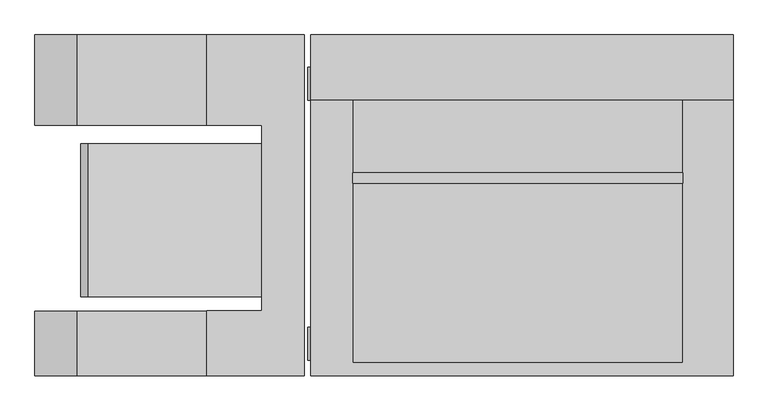
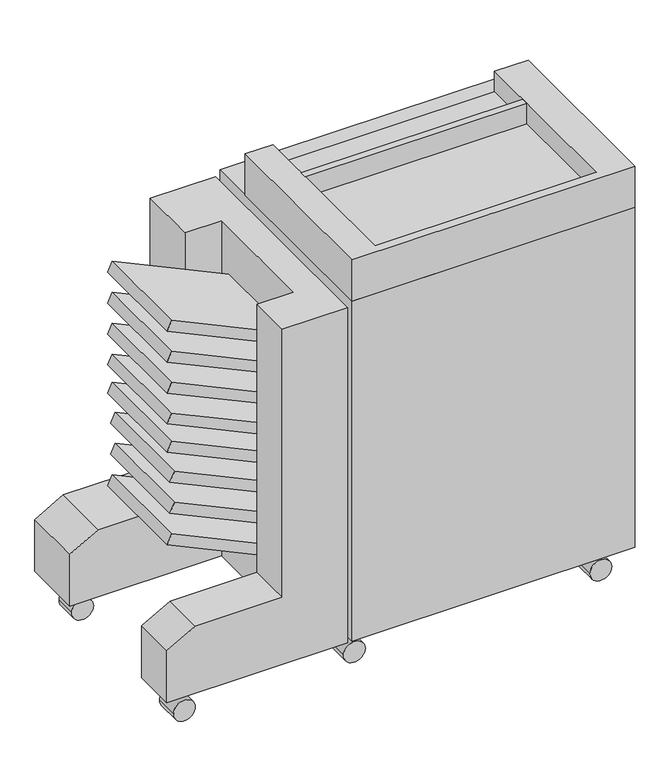
"""IFC4 building model written with IfcOpenShell, lengths in millimetres: proxy geometry, Kopierer : Kopierer."""

from ifc_helpers import new_model, si_unit, point, frame, frame_2d, origin, place, context, project, spatial, polyline, circle_curve, trimmed, segment, composite_curve, outline, extrude, faceted_brep, source, transform, mapped, element, save


def specialty_equipment_65fc0428(model_context):
    return source(origin(), model_context, "Body", "SolidModel", [
        extrude(outline(polyline([(387.7567294, -681.6535349), (364.7365116, -692.3880388), (232.9041289, -409.6725817), (260.929928, -409.6725817), (387.7567294, -681.6535349)])), frame((0.0, -167.6536807, 0.0), z_axis=(0.0, 1.0, 0.0), x_axis=(0.0, 0.0, 1.0)), (0.0, 0.0, 1.0), 239.8222339),
        extrude(outline(polyline([(463.6667654, -675.0122673), (440.6465476, -685.7467712), (311.9110388, -409.6725817), (339.9368379, -409.6725817), (463.6667654, -675.0122673)])), frame((0.0, -167.6536807, 0.0), z_axis=(0.0, 1.0, 0.0), x_axis=(0.0, 0.0, 1.0)), (0.0, 0.0, 1.0), 239.8222339),
        extrude(outline(polyline([(539.8667654, -675.0122673), (516.8465476, -685.7467712), (388.1110388, -409.6725817), (416.1368379, -409.6725817), (539.8667654, -675.0122673)])), frame((0.0, -167.6536807, 0.0), z_axis=(0.0, 1.0, 0.0), x_axis=(0.0, 0.0, 1.0)), (0.0, 0.0, 1.0), 239.8222339),
        extrude(outline(polyline([(914.2268014, -681.6535349), (891.2065836, -692.3880388), (759.3742009, -409.6725817), (787.4, -409.6725817), (914.2268014, -681.6535349)])), frame((0.0, -167.6536807, 0.0), z_axis=(0.0, 1.0, 0.0), x_axis=(0.0, 0.0, 1.0)), (0.0, 0.0, 1.0), 239.8222339),
        extrude(outline(polyline([(838.0268014, -681.6535349), (815.0065836, -692.3880388), (683.1742009, -409.6725817), (711.2, -409.6725817), (838.0268014, -681.6535349)])), frame((0.0, -167.6536807, 0.0), z_axis=(0.0, 1.0, 0.0), x_axis=(0.0, 0.0, 1.0)), (0.0, 0.0, 1.0), 239.8222339),
        extrude(outline(polyline([(615.7768014, -681.6535349), (592.7565836, -692.3880388), (460.9242009, -409.6725817), (488.95, -409.6725817), (615.7768014, -681.6535349)])), frame((0.0, -167.6536807, 0.0), z_axis=(0.0, 1.0, 0.0), x_axis=(0.0, 0.0, 1.0)), (0.0, 0.0, 1.0), 239.8222339),
        extrude(outline(polyline([(685.6268014, -681.6535349), (662.6065836, -692.3880388), (530.7742009, -409.6725817), (558.8, -409.6725817), (685.6268014, -681.6535349)])), frame((0.0, -167.6536807, 0.0), z_axis=(0.0, 1.0, 0.0), x_axis=(0.0, 0.0, 1.0)), (0.0, 0.0, 1.0), 239.8222339),
        extrude(outline(polyline([(761.8268014, -681.6535349), (738.8065836, -692.3880388), (606.9742009, -409.6725817), (635.0, -409.6725817), (761.8268014, -681.6535349)])), frame((0.0, -167.6536807, 0.0), z_axis=(0.0, 1.0, 0.0), x_axis=(0.0, 0.0, 1.0)), (0.0, 0.0, 1.0), 239.8222339),
        extrude(outline(composite_curve([segment(trimmed(circle_curve(frame_2d((26.0668925, -711.8709821)), 25.4), [point((26.0668925, -737.2709821))], [point((26.0668925, -686.4709821))], False, "CARTESIAN"), True, "CONTINUOUS"), segment(trimmed(circle_curve(frame_2d((26.0668925, -711.8709821)), 25.4), [point((26.0668925, -686.4709821))], [point((26.0668925, -737.2709821))], False, "CARTESIAN"), True, "CONTINUOUS")], self_intersect=False)), frame((0.0, -271.1108348, 0.0), z_axis=(0.0, 1.0, 0.0), x_axis=(0.0, 0.0, 1.0)), (0.0, 0.0, 1.0), 55.9418879),
        extrude(outline(composite_curve([segment(trimmed(circle_curve(frame_2d((26.0668925, -711.8709821)), 25.4), [point((26.0668925, -737.2709821))], [point((26.0668925, -686.4709821))], False, "CARTESIAN"), True, "CONTINUOUS"), segment(trimmed(circle_curve(frame_2d((26.0668925, -711.8709821)), 25.4), [point((26.0668925, -686.4709821))], [point((26.0668925, -737.2709821))], False, "CARTESIAN"), True, "CONTINUOUS")], self_intersect=False)), frame((0.0, 139.9052479, 0.0), z_axis=(0.0, 1.0, 0.0), x_axis=(0.0, 0.0, 1.0)), (0.0, 0.0, 1.0), 51.3258053),
        faceted_brep([(-764.1654582, 242.0310532, 76.2), (-764.1654582, 242.0310532, 203.2), (-698.1743224, 242.0310532, 241.3), (-494.9743224, 242.0310532, 241.3), (-494.9743224, 242.0310532, 901.7), (-342.5743224, 242.0310532, 901.7), (-342.5743224, 242.0310532, 76.2), (-764.1654582, -291.3689468, 76.2), (-342.5743224, -291.3689468, 76.2), (-342.5743224, -291.3689468, 901.7), (-494.9743224, -291.3689468, 901.7), (-494.9743224, -291.3689468, 241.3), (-698.1743224, -291.3689468, 241.3), (-764.1654582, -291.3689468, 203.2), (-764.1654582, -189.7689468, 76.2), (-409.6725817, -189.7689468, 76.2), (-409.6725817, 100.8888364, 76.2), (-764.1654582, 100.8888364, 76.2), (-494.9743224, 100.8888364, 901.7), (-409.6725817, 100.8888364, 901.7), (-409.6725817, -189.7689468, 901.7), (-494.9743224, -189.7689468, 901.7), (-494.9743224, -189.7689468, 241.3), (-494.9743224, 100.8888364, 241.3), (-698.1743224, -189.7689468, 241.3), (-698.1743224, 100.8888364, 241.3), (-764.1654582, -189.7689468, 203.2), (-764.1654582, 100.8888364, 203.2)], [[[0, 1, 2, 3, 4, 5, 6]], [[7, 8, 9, 10, 11, 12, 13]], [[6, 8, 7, 14, 15, 16, 17, 0]], [[5, 9, 8, 6]], [[4, 18, 19, 20, 21, 10, 9, 5]], [[10, 21, 22, 11]], [[3, 23, 18, 4]], [[11, 22, 24, 12]], [[2, 25, 23, 3]], [[12, 24, 26, 13]], [[1, 27, 25, 2]], [[0, 17, 27, 1]], [[13, 26, 14, 7]], [[15, 14, 26, 24, 22, 21, 20]], [[19, 18, 23, 25, 27, 17, 16]], [[20, 19, 16, 15]]]),
        extrude(outline(composite_curve([segment(trimmed(circle_curve(frame_2d((27.9129458, -312.2555429)), 25.4), [point((27.9129458, -337.6555429))], [point((27.9129458, -286.8555429))], False, "CARTESIAN"), True, "CONTINUOUS"), segment(trimmed(circle_curve(frame_2d((27.9129458, -312.2555429)), 25.4), [point((27.9129458, -286.8555429))], [point((27.9129458, -337.6555429))], False, "CARTESIAN"), True, "CONTINUOUS")], self_intersect=False)), frame((0.0, -266.4947521, 0.0), z_axis=(0.0, 1.0, 0.0), x_axis=(0.0, 0.0, 1.0)), (0.0, 0.0, 1.0), 51.3258053),
        extrude(outline(composite_curve([segment(trimmed(circle_curve(frame_2d((27.9129458, 262.7398948)), 25.4), [point((27.9129458, 237.3398948))], [point((27.9129458, 288.1398948))], False, "CARTESIAN"), True, "CONTINUOUS"), segment(trimmed(circle_curve(frame_2d((27.9129458, 262.7398948)), 25.4), [point((27.9129458, 288.1398948))], [point((27.9129458, 237.3398948))], False, "CARTESIAN"), True, "CONTINUOUS")], self_intersect=False)), frame((0.0, -266.4947521, 0.0), z_axis=(0.0, 1.0, 0.0), x_axis=(0.0, 0.0, 1.0)), (0.0, 0.0, 1.0), 51.3258053),
        extrude(outline(composite_curve([segment(trimmed(circle_curve(frame_2d((27.9129458, -312.2555429)), 25.4), [point((27.9129458, -337.6555429))], [point((27.9129458, -286.8555429))], False, "CARTESIAN"), True, "CONTINUOUS"), segment(trimmed(circle_curve(frame_2d((27.9129458, -312.2555429)), 25.4), [point((27.9129458, -286.8555429))], [point((27.9129458, -337.6555429))], False, "CARTESIAN"), True, "CONTINUOUS")], self_intersect=False)), frame((0.0, 139.9052479, 0.0), z_axis=(0.0, 1.0, 0.0), x_axis=(0.0, 0.0, 1.0)), (0.0, 0.0, 1.0), 51.3258053),
        extrude(outline(composite_curve([segment(trimmed(circle_curve(frame_2d((27.9129458, 262.7398948)), 25.4), [point((27.9129458, 237.3398948))], [point((27.9129458, 288.1398948))], False, "CARTESIAN"), True, "CONTINUOUS"), segment(trimmed(circle_curve(frame_2d((27.9129458, 262.7398948)), 25.4), [point((27.9129458, 288.1398948))], [point((27.9129458, 237.3398948))], False, "CARTESIAN"), True, "CONTINUOUS")], self_intersect=False)), frame((0.0, 139.9052479, 0.0), z_axis=(0.0, 1.0, 0.0), x_axis=(0.0, 0.0, 1.0)), (0.0, 0.0, 1.0), 51.3258053),
        extrude(outline(polyline([(249.314028, 26.1310532), (249.314028, 10.0577181), (-267.2959958, 10.0577181), (-267.2959958, 26.1310532), (249.314028, 26.1310532)])), frame((0.0, 0.0, 965.2), z_axis=(0.0, 0.0, 1.0), x_axis=(1.0, 0.0, 0.0)), (0.0, 0.0, 1.0), 50.8),
        faceted_brep([(249.314028, 242.0310532, 472.3553727), (-284.085972, 242.0310532, 472.3553727), (-284.085972, 242.0310532, 609.6), (249.314028, 242.0310532, 609.6), (-66.7741493, 242.0310532, 578.8591447), (-66.7741493, 242.0310532, 553.4591447), (34.8258507, 242.0310532, 553.4591447), (34.8258507, 242.0310532, 578.8591447), (249.314028, 191.2310532, 472.3553727), (249.314028, 191.2310532, 609.6), (-284.085972, 191.2310532, 609.6), (-284.085972, 191.2310532, 472.3553727), (34.8258507, 216.6310532, 578.8591447), (34.8258507, 216.6310532, 553.4591447), (-66.7741493, 216.6310532, 553.4591447), (-66.7741493, 216.6310532, 578.8591447)], [[[0, 1, 2, 3], [4, 5, 6, 7]], [[8, 9, 10, 11]], [[3, 9, 8, 0]], [[2, 10, 9, 3]], [[1, 11, 10, 2]], [[0, 8, 11, 1]], [[12, 13, 14, 15]], [[15, 4, 7, 12]], [[14, 5, 4, 15]], [[13, 6, 5, 14]], [[12, 7, 6, 13]]]),
        faceted_brep([(249.314028, 242.0310532, 283.8723489), (-284.085972, 242.0310532, 283.8723489), (-284.085972, 242.0310532, 472.3553727), (249.314028, 242.0310532, 472.3553727), (-66.7741493, 242.0310532, 432.3774172), (-66.7741493, 242.0310532, 406.4), (34.8258507, 242.0310532, 406.4), (34.8258507, 242.0310532, 432.3774172), (249.314028, 191.2310532, 283.8723489), (249.314028, 191.2310532, 472.3553727), (-284.085972, 191.2310532, 472.3553727), (-284.085972, 191.2310532, 283.8723489), (34.8258507, 216.6310532, 432.3774172), (34.8258507, 216.6310532, 406.4), (-66.7741493, 216.6310532, 406.4), (-66.7741493, 216.6310532, 432.3774172)], [[[0, 1, 2, 3], [4, 5, 6, 7]], [[8, 9, 10, 11]], [[3, 9, 8, 0]], [[2, 10, 9, 3]], [[1, 11, 10, 2]], [[0, 8, 11, 1]], [[12, 13, 14, 15]], [[15, 4, 7, 12]], [[14, 5, 4, 15]], [[13, 6, 5, 14]], [[12, 7, 6, 13]]]),
        faceted_brep([(249.314028, 242.0310532, 76.2), (-284.085972, 242.0310532, 76.2), (-284.085972, 242.0310532, 283.8723489), (249.314028, 242.0310532, 283.8723489), (-66.7741493, 242.0310532, 246.5423898), (-66.7741493, 242.0310532, 211.1096445), (34.8258507, 242.0310532, 211.1096445), (34.8258507, 242.0310532, 246.5423898), (249.314028, 191.2310532, 76.2), (249.314028, 191.2310532, 283.8723489), (-284.085972, 191.2310532, 283.8723489), (-284.085972, 191.2310532, 76.2), (34.8258507, 216.6310532, 246.5423898), (34.8258507, 216.6310532, 211.1096445), (-66.7741493, 216.6310532, 211.1096445), (-66.7741493, 216.6310532, 246.5423898)], [[[0, 1, 2, 3], [4, 5, 6, 7]], [[8, 9, 10, 11]], [[3, 9, 8, 0]], [[2, 10, 9, 3]], [[1, 11, 10, 2]], [[0, 8, 11, 1]], [[12, 13, 14, 15]], [[15, 4, 7, 12]], [[14, 5, 4, 15]], [[13, 6, 5, 14]], [[12, 7, 6, 13]]]),
        faceted_brep([(328.0345418, -291.3689468, 1016.0), (328.0345418, 139.9052479, 1016.0), (249.314028, 139.9052479, 1016.0), (249.314028, -271.1108348, 1016.0), (-267.2959958, -271.1108348, 1016.0), (-267.2959958, 139.9052479, 1016.0), (-332.3654582, 139.9052479, 1016.0), (-332.3654582, -291.3689468, 1016.0), (328.0345418, -291.3689468, 914.4), (-332.3654582, -291.3689468, 914.4), (-332.3654582, 139.9052479, 914.4), (328.0345418, 139.9052479, 914.4), (-267.2959958, 139.9052479, 965.2), (249.314028, 139.9052479, 965.2), (249.314028, -271.1108348, 965.2), (-267.2959958, -271.1108348, 965.2)], [[[0, 1, 2, 3, 4, 5, 6, 7]], [[8, 9, 10, 11]], [[7, 9, 8, 0]], [[6, 10, 9, 7]], [[10, 6, 5, 12, 13, 2, 1, 11]], [[0, 8, 11, 1]], [[14, 13, 12, 15]], [[15, 4, 3, 14]], [[12, 5, 4, 15]], [[14, 3, 2, 13]]]),
        faceted_brep([(328.0345418, -291.3689468, 914.4), (328.0345418, 242.0310532, 914.4), (-332.3654582, 242.0310532, 914.4), (-332.3654582, -291.3689468, 914.4), (328.0345418, -291.3689468, 76.2), (-332.3654582, -291.3689468, 76.2), (-332.3654582, 242.0310532, 76.2), (-284.085972, 242.0310532, 76.2), (-284.085972, 191.2310532, 76.2), (249.314028, 191.2310532, 76.2), (249.314028, 242.0310532, 76.2), (328.0345418, 242.0310532, 76.2), (249.314028, 242.0310532, 609.6), (-284.085972, 242.0310532, 609.6), (-284.085972, 191.2310532, 609.6), (249.314028, 191.2310532, 609.6)], [[[0, 1, 2, 3]], [[4, 5, 6, 7, 8, 9, 10, 11]], [[3, 5, 4, 0]], [[2, 6, 5, 3]], [[1, 11, 10, 12, 13, 7, 6, 2]], [[0, 4, 11, 1]], [[14, 15, 9, 8]], [[8, 7, 13, 14]], [[15, 12, 10, 9]], [[14, 13, 12, 15]]]),
    ])


if __name__ == "__main__":
    model = new_model("IFC4")
    model_context = context("Model", 3, world=origin())
    ifc_project = project(units=[si_unit("LENGTHUNIT", "METRE", prefix="MILLI")], contexts=[model_context])
    site = spatial("IfcSite", under=ifc_project)
    building = spatial("IfcBuilding", under=site)
    placement = place(None, origin())
    specialty_equipment_shape = specialty_equipment_65fc0428(model_context)
    element("IfcBuildingElementProxy", 1, Name="Kopierer : Kopierer", ObjectType="Kopierer : Kopierer", at=placement, inside=building, context=model_context, shape_type="MappedRepresentation", body=[
        mapped(specialty_equipment_shape, transform((0.0, 0.0, 0.0), x_axis=(1.0, 0.0, 0.0), y_axis=(0.0, 1.0, 0.0), z_axis=(0.0, 0.0, 1.0))),
    ])
    save(model, "model.ifc")

# Revit data of these elements
# Type "Kopierer : Kopierer"
#   Assembly Code = ""
# Element 1 (IfcBuildingElementProxy, "Kopierer : Kopierer")
#   Materials on its faces: "Kunststoff - Weiß", "Kunststoff - grau, dunkel"
# Materials
#   "Kunststoff - Weiß": class "Kunststoff", colour RGB 249 249 249, transparency 0, Cost = 0
#   "Kunststoff - grau, dunkel": class "Kunststoff", colour RGB 134 134 134, transparency 0
